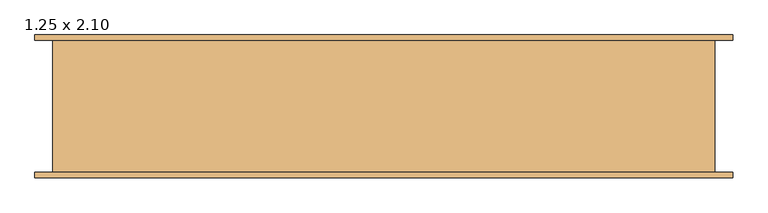
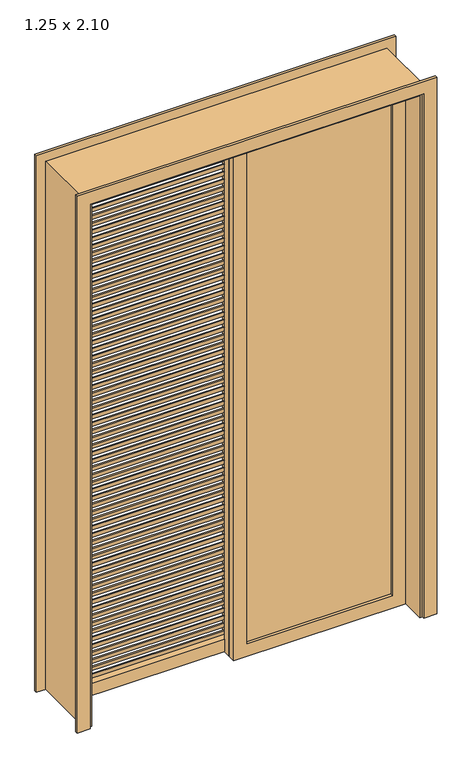
"""IFC4 building model written with IfcOpenShell, lengths in millimetres: door geometry, .CC_ND 300_PORTA DE CORRER_3 FOLHAS_VENEZIANA_VIDRO_COM EXTENSÃO : 1.25 x 2.10."""

import ifcopenshell
import ifcopenshell.guid

model = None  # the IFC model being written
_history = None  # IfcOwnerHistory: only IFC2X3 demands one
_inside = {}  # id of a spatial element -> (the spatial element, [elements in it])
_under = {}  # id of a project, library or spatial element -> (it, [spatial elements below it])
_declared = {}  # id of a project -> (the project, [libraries it declares])
_typed = {}  # id of a type object -> (the type object, [elements of that type])
_made_of = {}  # id of a material, layer set ... -> (it, [elements and type objects made of it])


def new_model(schema):
    """Start an empty IFC model of exactly this schema.

    Asked for "IFC4X3", IfcOpenShell would pick the latest addendum, in which some entities
    have other attributes; the version numbers below select the first issue.
    IFC2X3 requires an IfcOwnerHistory on every rooted entity: one is made here for all.
    """
    global model, _history
    if schema == "IFC4X3":
        model = ifcopenshell.file(schema_version=(4, 3, 0, 0))
    else:
        model = ifcopenshell.file(schema=schema)
    _inside.clear()
    _under.clear()
    _declared.clear()
    _typed.clear()
    _made_of.clear()
    _history = None
    if model.schema == "IFC2X3":
        org = make("IfcOrganization", Name="unknown")
        user = make(
            "IfcPersonAndOrganization",
            ThePerson=make("IfcPerson", FamilyName="unknown"),
            TheOrganization=org,
        )
        app = make(
            "IfcApplication",
            ApplicationDeveloper=org,
            Version="unknown",
            ApplicationFullName="unknown",
            ApplicationIdentifier="unknown",
        )
        _history = make(
            "IfcOwnerHistory",
            OwningUser=user,
            OwningApplication=app,
            ChangeAction="ADDED",
            CreationDate=0,
        )
    return model


def make(cls, **values):
    """One entity of the class cls with the attributes given. An attribute that is None is left unset."""
    return model.create_entity(
        cls, **{name: value for name, value in values.items() if value is not None}
    )


def rooted(cls, **values):
    """An entity with a GlobalId (a new one), such as an element, a storey or a relation."""
    return make(cls, GlobalId=ifcopenshell.guid.new(), OwnerHistory=_history, **values)


def si_unit(unit_type, name, prefix=None):
    """IfcSIUnit, for example si_unit("LENGTHUNIT", "METRE", prefix="MILLI")."""
    return make("IfcSIUnit", UnitType=unit_type, Prefix=prefix, Name=name)


def assignment(units):
    """IfcUnitAssignment: the units of a project."""
    return None if units is None else make("IfcUnitAssignment", Units=units)


def point(xyz):
    """IfcCartesianPoint."""
    return None if xyz is None else make("IfcCartesianPoint", Coordinates=xyz)


def direction(xyz):
    """IfcDirection."""
    return None if xyz is None else make("IfcDirection", DirectionRatios=xyz)


def frame(location, z_axis=None, x_axis=None):
    """IfcAxis2Placement3D, a coordinate frame: its origin and axes. An axis left out is left unset."""
    return make(
        "IfcAxis2Placement3D",
        Location=point(location),
        Axis=direction(z_axis),
        RefDirection=direction(x_axis),
    )


def origin():
    """The frame at (0, 0, 0) with its axes left unset."""
    return frame((0.0, 0.0, 0.0))


def place(relative_to, where):
    """IfcLocalPlacement: puts the frame where relative to a parent placement (None: the world)."""
    return make(
        "IfcLocalPlacement", PlacementRelTo=relative_to, RelativePlacement=where
    )


def context(
    kind, dimensions, precision=None, world=None, true_north=None, identifier=None
):
    """IfcGeometricRepresentationContext, for example the 3D "Model" context."""
    return make(
        "IfcGeometricRepresentationContext",
        ContextIdentifier=identifier,
        ContextType=kind,
        CoordinateSpaceDimension=dimensions,
        Precision=precision,
        WorldCoordinateSystem=world,
        TrueNorth=true_north,
    )


def project(units=None, contexts=None):
    """IfcProject with its units and contexts."""
    return rooted(
        "IfcProject",
        Name="project",
        RepresentationContexts=contexts,
        UnitsInContext=assignment(units),
    )


def spatial(cls, under=None, at=None, **own):
    """A site, building, storey or space (cls), placed at a placement, below another one or the project."""
    s = rooted(cls, ObjectPlacement=at, **own)
    if under is not None:
        _under.setdefault(under.id(), (under, []))[1].append(s)
    return s


def polyline(points):
    """IfcPolyline through the points."""
    return make("IfcPolyline", Points=[point(p) for p in points])


def outline(outer, holes=None, kind="AREA"):
    """IfcArbitraryClosedProfileDef: a profile drawn as a closed curve; with holes, ...WithVoids."""
    if holes is None:
        return make("IfcArbitraryClosedProfileDef", ProfileType=kind, OuterCurve=outer)
    return make(
        "IfcArbitraryProfileDefWithVoids",
        ProfileType=kind,
        OuterCurve=outer,
        InnerCurves=holes,
    )


def extrude(swept, where, along, depth):
    """IfcExtrudedAreaSolid: the profile swept, set in the frame where, extruded along a direction by depth."""
    return make(
        "IfcExtrudedAreaSolid",
        SweptArea=swept,
        Position=where,
        ExtrudedDirection=direction(along),
        Depth=depth,
    )


def shape(context_of_items, identifier, shape_type, items):
    """IfcShapeRepresentation: the items that make up one representation, for example the "Body"."""
    return make(
        "IfcShapeRepresentation",
        ContextOfItems=context_of_items,
        RepresentationIdentifier=identifier,
        RepresentationType=shape_type,
        Items=items,
    )


def source(mapping_origin, context_of_items, identifier, shape_type, items):
    """IfcRepresentationMap: a shape defined once, which mapped items show again and again."""
    return make(
        "IfcRepresentationMap",
        MappingOrigin=mapping_origin,
        MappedRepresentation=shape(context_of_items, identifier, shape_type, items),
    )


def transform(
    local_origin,
    x_axis=None,
    y_axis=None,
    z_axis=None,
    scale=None,
    scale2=None,
    scale3=None,
    uniform=True,
):
    """IfcCartesianTransformationOperator3D, or its non-uniform kind. x_axis, y_axis, z_axis: its Axis1, 2, 3."""
    if uniform:
        return make(
            "IfcCartesianTransformationOperator3D",
            Axis1=direction(x_axis),
            Axis2=direction(y_axis),
            LocalOrigin=point(local_origin),
            Scale=scale,
            Axis3=direction(z_axis),
        )
    return make(
        "IfcCartesianTransformationOperator3DnonUniform",
        Axis1=direction(x_axis),
        Axis2=direction(y_axis),
        LocalOrigin=point(local_origin),
        Scale=scale,
        Axis3=direction(z_axis),
        Scale2=scale2,
        Scale3=scale3,
    )


def mapped(mapping_source, mapping_target):
    """IfcMappedItem: shows the shape of a source again, moved by a transform."""
    return make(
        "IfcMappedItem", MappingSource=mapping_source, MappingTarget=mapping_target
    )


def made_of(thing, what):
    """Note that an element or type object is made of a material, layer set ...; save() writes the relation."""
    if what is not None:
        _made_of.setdefault(what.id(), (what, []))[1].append(thing)
    return thing


def element(
    cls,
    number,
    at=None,
    inside=None,
    cuts=None,
    type_object=None,
    material=None,
    context=None,
    identifier="Body",
    shape_type=None,
    held_by="IfcProductDefinitionShape",
    body=None,
    shapes=None,
    **own,
):
    """One element of the class cls, such as IfcWall. Its Tag is "e" and its number.

    at: its placement. inside: the storey or other place that contains it. cuts: it is an
    opening in that element (IfcRelVoidsElement). A single representation is given by context,
    identifier, shape_type and body (its items); several are given by shapes. held_by: the class
    of the entity that holds the representations. save() writes the other relations.
    """
    e = rooted(cls, Tag="e%d" % number, ObjectPlacement=at, **own)
    if body is not None:
        shapes = [shape(context, identifier, shape_type, body)]
    if shapes is not None:
        e.Representation = make(held_by, Representations=shapes)
    if inside is not None:
        _inside.setdefault(inside.id(), (inside, []))[1].append(e)
    if cuts is not None:
        rooted(
            "IfcRelVoidsElement", RelatingBuildingElement=cuts, RelatedOpeningElement=e
        )
    if type_object is not None:
        _typed.setdefault(type_object.id(), (type_object, []))[1].append(e)
    return made_of(e, material)


def aggregate(whole, parts):
    """IfcRelAggregates: a whole, such as a stair, and the parts it consists of."""
    return rooted("IfcRelAggregates", RelatingObject=whole, RelatedObjects=parts)


def save(model, path):
    """Write the relations noted so far, then the file.

    IfcRelAggregates (storeys below a building ...), IfcRelContainedInSpatialStructure (elements
    in a storey), IfcRelDefinesByType, IfcRelAssociatesMaterial and IfcRelDeclares: one each for
    every whole, place, type object, material and project.
    """
    for whole, parts in _under.values():
        aggregate(whole, parts)
    for where, things in _inside.values():
        rooted(
            "IfcRelContainedInSpatialStructure",
            RelatedElements=things,
            RelatingStructure=where,
        )
    for kind, things in _typed.values():
        rooted("IfcRelDefinesByType", RelatedObjects=things, RelatingType=kind)
    for what, things in _made_of.values():
        rooted("IfcRelAssociatesMaterial", RelatedObjects=things, RelatingMaterial=what)
    for by, libraries in _declared.values():
        rooted("IfcRelDeclares", RelatingContext=by, RelatedDefinitions=libraries)
    model.write(path)


def door_1_25_x_2_10_d20a60c6(model_context):
    return source(origin(), model_context, "Body", "SweptSolid", [
        extrude(outline(polyline([(575.0, -26.0), (575.0, -34.0), (20.0, -34.0), (20.0, -26.0), (575.0, -26.0)])), frame((0.0, 0.0, 50.0), z_axis=(0.0, 0.0, 1.0), x_axis=(1.0, 0.0, 0.0)), (0.0, 0.0, 1.0), 2000.0),
        extrude(outline(polyline([(2100.0, 625.0), (2100.0, -30.0), (0.0, -30.0), (0.0, 625.0), (2100.0, 625.0)]), holes=[polyline([(2050.0, 575.0), (50.0, 575.0), (50.0, 20.0), (2050.0, 20.0), (2050.0, 575.0)])]), frame((0.0, -45.0, 0.0), z_axis=(0.0, 1.0, 0.0), x_axis=(0.0, 0.0, 1.0)), (0.0, 0.0, 1.0), 30.0),
        extrude(outline(polyline([(40.0, 1985.2272727), (15.0, 2020.2272727), (20.0, 2020.2272727), (45.0, 1985.2272727), (40.0, 1985.2272727)])), frame((-575.0, 0.0, 0.0), z_axis=(1.0, 0.0, 0.0), x_axis=(0.0, 1.0, 0.0)), (0.0, 0.0, 1.0), 555.0),
        extrude(outline(polyline([(40.0, 1955.4545455), (15.0, 1990.4545455), (20.0, 1990.4545455), (45.0, 1955.4545455), (40.0, 1955.4545455)])), frame((-575.0, 0.0, 0.0), z_axis=(1.0, 0.0, 0.0), x_axis=(0.0, 1.0, 0.0)), (0.0, 0.0, 1.0), 555.0),
        extrude(outline(polyline([(40.0, 1925.6818182), (15.0, 1960.6818182), (20.0, 1960.6818182), (45.0, 1925.6818182), (40.0, 1925.6818182)])), frame((-575.0, 0.0, 0.0), z_axis=(1.0, 0.0, 0.0), x_axis=(0.0, 1.0, 0.0)), (0.0, 0.0, 1.0), 555.0),
        extrude(outline(polyline([(40.0, 1895.9090909), (15.0, 1930.9090909), (20.0, 1930.9090909), (45.0, 1895.9090909), (40.0, 1895.9090909)])), frame((-575.0, 0.0, 0.0), z_axis=(1.0, 0.0, 0.0), x_axis=(0.0, 1.0, 0.0)), (0.0, 0.0, 1.0), 555.0),
        extrude(outline(polyline([(40.0, 1866.1363636), (15.0, 1901.1363636), (20.0, 1901.1363636), (45.0, 1866.1363636), (40.0, 1866.1363636)])), frame((-575.0, 0.0, 0.0), z_axis=(1.0, 0.0, 0.0), x_axis=(0.0, 1.0, 0.0)), (0.0, 0.0, 1.0), 555.0),
        extrude(outline(polyline([(40.0, 1836.3636364), (15.0, 1871.3636364), (20.0, 1871.3636364), (45.0, 1836.3636364), (40.0, 1836.3636364)])), frame((-575.0, 0.0, 0.0), z_axis=(1.0, 0.0, 0.0), x_axis=(0.0, 1.0, 0.0)), (0.0, 0.0, 1.0), 555.0),
        extrude(outline(polyline([(40.0, 1806.5909091), (15.0, 1841.5909091), (20.0, 1841.5909091), (45.0, 1806.5909091), (40.0, 1806.5909091)])), frame((-575.0, 0.0, 0.0), z_axis=(1.0, 0.0, 0.0), x_axis=(0.0, 1.0, 0.0)), (0.0, 0.0, 1.0), 555.0),
        extrude(outline(polyline([(40.0, 1776.8181818), (15.0, 1811.8181818), (20.0, 1811.8181818), (45.0, 1776.8181818), (40.0, 1776.8181818)])), frame((-575.0, 0.0, 0.0), z_axis=(1.0, 0.0, 0.0), x_axis=(0.0, 1.0, 0.0)), (0.0, 0.0, 1.0), 555.0),
        extrude(outline(polyline([(40.0, 1747.0454545), (15.0, 1782.0454545), (20.0, 1782.0454545), (45.0, 1747.0454545), (40.0, 1747.0454545)])), frame((-575.0, 0.0, 0.0), z_axis=(1.0, 0.0, 0.0), x_axis=(0.0, 1.0, 0.0)), (0.0, 0.0, 1.0), 555.0),
        extrude(outline(polyline([(40.0, 1717.2727273), (15.0, 1752.2727273), (20.0, 1752.2727273), (45.0, 1717.2727273), (40.0, 1717.2727273)])), frame((-575.0, 0.0, 0.0), z_axis=(1.0, 0.0, 0.0), x_axis=(0.0, 1.0, 0.0)), (0.0, 0.0, 1.0), 555.0),
        extrude(outline(polyline([(40.0, 1687.5), (15.0, 1722.5), (20.0, 1722.5), (45.0, 1687.5), (40.0, 1687.5)])), frame((-575.0, 0.0, 0.0), z_axis=(1.0, 0.0, 0.0), x_axis=(0.0, 1.0, 0.0)), (0.0, 0.0, 1.0), 555.0),
        extrude(outline(polyline([(40.0, 1657.7272727), (15.0, 1692.7272727), (20.0, 1692.7272727), (45.0, 1657.7272727), (40.0, 1657.7272727)])), frame((-575.0, 0.0, 0.0), z_axis=(1.0, 0.0, 0.0), x_axis=(0.0, 1.0, 0.0)), (0.0, 0.0, 1.0), 555.0),
        extrude(outline(polyline([(40.0, 1627.9545455), (15.0, 1662.9545455), (20.0, 1662.9545455), (45.0, 1627.9545455), (40.0, 1627.9545455)])), frame((-575.0, 0.0, 0.0), z_axis=(1.0, 0.0, 0.0), x_axis=(0.0, 1.0, 0.0)), (0.0, 0.0, 1.0), 555.0),
        extrude(outline(polyline([(40.0, 1598.1818182), (15.0, 1633.1818182), (20.0, 1633.1818182), (45.0, 1598.1818182), (40.0, 1598.1818182)])), frame((-575.0, 0.0, 0.0), z_axis=(1.0, 0.0, 0.0), x_axis=(0.0, 1.0, 0.0)), (0.0, 0.0, 1.0), 555.0),
        extrude(outline(polyline([(40.0, 1568.4090909), (15.0, 1603.4090909), (20.0, 1603.4090909), (45.0, 1568.4090909), (40.0, 1568.4090909)])), frame((-575.0, 0.0, 0.0), z_axis=(1.0, 0.0, 0.0), x_axis=(0.0, 1.0, 0.0)), (0.0, 0.0, 1.0), 555.0),
        extrude(outline(polyline([(40.0, 1538.6363636), (15.0, 1573.6363636), (20.0, 1573.6363636), (45.0, 1538.6363636), (40.0, 1538.6363636)])), frame((-575.0, 0.0, 0.0), z_axis=(1.0, 0.0, 0.0), x_axis=(0.0, 1.0, 0.0)), (0.0, 0.0, 1.0), 555.0),
        extrude(outline(polyline([(40.0, 1508.8636364), (15.0, 1543.8636364), (20.0, 1543.8636364), (45.0, 1508.8636364), (40.0, 1508.8636364)])), frame((-575.0, 0.0, 0.0), z_axis=(1.0, 0.0, 0.0), x_axis=(0.0, 1.0, 0.0)), (0.0, 0.0, 1.0), 555.0),
        extrude(outline(polyline([(40.0, 1479.0909091), (15.0, 1514.0909091), (20.0, 1514.0909091), (45.0, 1479.0909091), (40.0, 1479.0909091)])), frame((-575.0, 0.0, 0.0), z_axis=(1.0, 0.0, 0.0), x_axis=(0.0, 1.0, 0.0)), (0.0, 0.0, 1.0), 555.0),
        extrude(outline(polyline([(40.0, 1449.3181818), (15.0, 1484.3181818), (20.0, 1484.3181818), (45.0, 1449.3181818), (40.0, 1449.3181818)])), frame((-575.0, 0.0, 0.0), z_axis=(1.0, 0.0, 0.0), x_axis=(0.0, 1.0, 0.0)), (0.0, 0.0, 1.0), 555.0),
        extrude(outline(polyline([(40.0, 1419.5454545), (15.0, 1454.5454545), (20.0, 1454.5454545), (45.0, 1419.5454545), (40.0, 1419.5454545)])), frame((-575.0, 0.0, 0.0), z_axis=(1.0, 0.0, 0.0), x_axis=(0.0, 1.0, 0.0)), (0.0, 0.0, 1.0), 555.0),
        extrude(outline(polyline([(40.0, 1389.7727273), (15.0, 1424.7727273), (20.0, 1424.7727273), (45.0, 1389.7727273), (40.0, 1389.7727273)])), frame((-575.0, 0.0, 0.0), z_axis=(1.0, 0.0, 0.0), x_axis=(0.0, 1.0, 0.0)), (0.0, 0.0, 1.0), 555.0),
        extrude(outline(polyline([(40.0, 1360.0), (15.0, 1395.0), (20.0, 1395.0), (45.0, 1360.0), (40.0, 1360.0)])), frame((-575.0, 0.0, 0.0), z_axis=(1.0, 0.0, 0.0), x_axis=(0.0, 1.0, 0.0)), (0.0, 0.0, 1.0), 555.0),
        extrude(outline(polyline([(40.0, 1330.2272727), (15.0, 1365.2272727), (20.0, 1365.2272727), (45.0, 1330.2272727), (40.0, 1330.2272727)])), frame((-575.0, 0.0, 0.0), z_axis=(1.0, 0.0, 0.0), x_axis=(0.0, 1.0, 0.0)), (0.0, 0.0, 1.0), 555.0),
        extrude(outline(polyline([(40.0, 1300.4545455), (15.0, 1335.4545455), (20.0, 1335.4545455), (45.0, 1300.4545455), (40.0, 1300.4545455)])), frame((-575.0, 0.0, 0.0), z_axis=(1.0, 0.0, 0.0), x_axis=(0.0, 1.0, 0.0)), (0.0, 0.0, 1.0), 555.0),
        extrude(outline(polyline([(40.0, 1270.6818182), (15.0, 1305.6818182), (20.0, 1305.6818182), (45.0, 1270.6818182), (40.0, 1270.6818182)])), frame((-575.0, 0.0, 0.0), z_axis=(1.0, 0.0, 0.0), x_axis=(0.0, 1.0, 0.0)), (0.0, 0.0, 1.0), 555.0),
        extrude(outline(polyline([(40.0, 1240.9090909), (15.0, 1275.9090909), (20.0, 1275.9090909), (45.0, 1240.9090909), (40.0, 1240.9090909)])), frame((-575.0, 0.0, 0.0), z_axis=(1.0, 0.0, 0.0), x_axis=(0.0, 1.0, 0.0)), (0.0, 0.0, 1.0), 555.0),
        extrude(outline(polyline([(40.0, 1211.1363636), (15.0, 1246.1363636), (20.0, 1246.1363636), (45.0, 1211.1363636), (40.0, 1211.1363636)])), frame((-575.0, 0.0, 0.0), z_axis=(1.0, 0.0, 0.0), x_axis=(0.0, 1.0, 0.0)), (0.0, 0.0, 1.0), 555.0),
        extrude(outline(polyline([(40.0, 1181.3636364), (15.0, 1216.3636364), (20.0, 1216.3636364), (45.0, 1181.3636364), (40.0, 1181.3636364)])), frame((-575.0, 0.0, 0.0), z_axis=(1.0, 0.0, 0.0), x_axis=(0.0, 1.0, 0.0)), (0.0, 0.0, 1.0), 555.0),
        extrude(outline(polyline([(40.0, 1151.5909091), (15.0, 1186.5909091), (20.0, 1186.5909091), (45.0, 1151.5909091), (40.0, 1151.5909091)])), frame((-575.0, 0.0, 0.0), z_axis=(1.0, 0.0, 0.0), x_axis=(0.0, 1.0, 0.0)), (0.0, 0.0, 1.0), 555.0),
        extrude(outline(polyline([(40.0, 1121.8181818), (15.0, 1156.8181818), (20.0, 1156.8181818), (45.0, 1121.8181818), (40.0, 1121.8181818)])), frame((-575.0, 0.0, 0.0), z_axis=(1.0, 0.0, 0.0), x_axis=(0.0, 1.0, 0.0)), (0.0, 0.0, 1.0), 555.0),
        extrude(outline(polyline([(40.0, 1092.0454545), (15.0, 1127.0454545), (20.0, 1127.0454545), (45.0, 1092.0454545), (40.0, 1092.0454545)])), frame((-575.0, 0.0, 0.0), z_axis=(1.0, 0.0, 0.0), x_axis=(0.0, 1.0, 0.0)), (0.0, 0.0, 1.0), 555.0),
        extrude(outline(polyline([(40.0, 1062.2727273), (15.0, 1097.2727273), (20.0, 1097.2727273), (45.0, 1062.2727273), (40.0, 1062.2727273)])), frame((-575.0, 0.0, 0.0), z_axis=(1.0, 0.0, 0.0), x_axis=(0.0, 1.0, 0.0)), (0.0, 0.0, 1.0), 555.0),
        extrude(outline(polyline([(40.0, 1032.5), (15.0, 1067.5), (20.0, 1067.5), (45.0, 1032.5), (40.0, 1032.5)])), frame((-575.0, 0.0, 0.0), z_axis=(1.0, 0.0, 0.0), x_axis=(0.0, 1.0, 0.0)), (0.0, 0.0, 1.0), 555.0),
        extrude(outline(polyline([(40.0, 1002.7272727), (15.0, 1037.7272727), (20.0, 1037.7272727), (45.0, 1002.7272727), (40.0, 1002.7272727)])), frame((-575.0, 0.0, 0.0), z_axis=(1.0, 0.0, 0.0), x_axis=(0.0, 1.0, 0.0)), (0.0, 0.0, 1.0), 555.0),
        extrude(outline(polyline([(40.0, 972.9545455), (15.0, 1007.9545455), (20.0, 1007.9545455), (45.0, 972.9545455), (40.0, 972.9545455)])), frame((-575.0, 0.0, 0.0), z_axis=(1.0, 0.0, 0.0), x_axis=(0.0, 1.0, 0.0)), (0.0, 0.0, 1.0), 555.0),
        extrude(outline(polyline([(40.0, 943.1818182), (15.0, 978.1818182), (20.0, 978.1818182), (45.0, 943.1818182), (40.0, 943.1818182)])), frame((-575.0, 0.0, 0.0), z_axis=(1.0, 0.0, 0.0), x_axis=(0.0, 1.0, 0.0)), (0.0, 0.0, 1.0), 555.0),
        extrude(outline(polyline([(40.0, 913.4090909), (15.0, 948.4090909), (20.0, 948.4090909), (45.0, 913.4090909), (40.0, 913.4090909)])), frame((-575.0, 0.0, 0.0), z_axis=(1.0, 0.0, 0.0), x_axis=(0.0, 1.0, 0.0)), (0.0, 0.0, 1.0), 555.0),
        extrude(outline(polyline([(40.0, 883.6363636), (15.0, 918.6363636), (20.0, 918.6363636), (45.0, 883.6363636), (40.0, 883.6363636)])), frame((-575.0, 0.0, 0.0), z_axis=(1.0, 0.0, 0.0), x_axis=(0.0, 1.0, 0.0)), (0.0, 0.0, 1.0), 555.0),
        extrude(outline(polyline([(40.0, 853.8636364), (15.0, 888.8636364), (20.0, 888.8636364), (45.0, 853.8636364), (40.0, 853.8636364)])), frame((-575.0, 0.0, 0.0), z_axis=(1.0, 0.0, 0.0), x_axis=(0.0, 1.0, 0.0)), (0.0, 0.0, 1.0), 555.0),
        extrude(outline(polyline([(40.0, 824.0909091), (15.0, 859.0909091), (20.0, 859.0909091), (45.0, 824.0909091), (40.0, 824.0909091)])), frame((-575.0, 0.0, 0.0), z_axis=(1.0, 0.0, 0.0), x_axis=(0.0, 1.0, 0.0)), (0.0, 0.0, 1.0), 555.0),
        extrude(outline(polyline([(40.0, 794.3181818), (15.0, 829.3181818), (20.0, 829.3181818), (45.0, 794.3181818), (40.0, 794.3181818)])), frame((-575.0, 0.0, 0.0), z_axis=(1.0, 0.0, 0.0), x_axis=(0.0, 1.0, 0.0)), (0.0, 0.0, 1.0), 555.0),
        extrude(outline(polyline([(40.0, 764.5454545), (15.0, 799.5454545), (20.0, 799.5454545), (45.0, 764.5454545), (40.0, 764.5454545)])), frame((-575.0, 0.0, 0.0), z_axis=(1.0, 0.0, 0.0), x_axis=(0.0, 1.0, 0.0)), (0.0, 0.0, 1.0), 555.0),
        extrude(outline(polyline([(40.0, 734.7727273), (15.0, 769.7727273), (20.0, 769.7727273), (45.0, 734.7727273), (40.0, 734.7727273)])), frame((-575.0, 0.0, 0.0), z_axis=(1.0, 0.0, 0.0), x_axis=(0.0, 1.0, 0.0)), (0.0, 0.0, 1.0), 555.0),
        extrude(outline(polyline([(40.0, 705.0), (15.0, 740.0), (20.0, 740.0), (45.0, 705.0), (40.0, 705.0)])), frame((-575.0, 0.0, 0.0), z_axis=(1.0, 0.0, 0.0), x_axis=(0.0, 1.0, 0.0)), (0.0, 0.0, 1.0), 555.0),
        extrude(outline(polyline([(40.0, 675.2272727), (15.0, 710.2272727), (20.0, 710.2272727), (45.0, 675.2272727), (40.0, 675.2272727)])), frame((-575.0, 0.0, 0.0), z_axis=(1.0, 0.0, 0.0), x_axis=(0.0, 1.0, 0.0)), (0.0, 0.0, 1.0), 555.0),
        extrude(outline(polyline([(40.0, 645.4545455), (15.0, 680.4545455), (20.0, 680.4545455), (45.0, 645.4545455), (40.0, 645.4545455)])), frame((-575.0, 0.0, 0.0), z_axis=(1.0, 0.0, 0.0), x_axis=(0.0, 1.0, 0.0)), (0.0, 0.0, 1.0), 555.0),
        extrude(outline(polyline([(40.0, 615.6818182), (15.0, 650.6818182), (20.0, 650.6818182), (45.0, 615.6818182), (40.0, 615.6818182)])), frame((-575.0, 0.0, 0.0), z_axis=(1.0, 0.0, 0.0), x_axis=(0.0, 1.0, 0.0)), (0.0, 0.0, 1.0), 555.0),
        extrude(outline(polyline([(40.0, 585.9090909), (15.0, 620.9090909), (20.0, 620.9090909), (45.0, 585.9090909), (40.0, 585.9090909)])), frame((-575.0, 0.0, 0.0), z_axis=(1.0, 0.0, 0.0), x_axis=(0.0, 1.0, 0.0)), (0.0, 0.0, 1.0), 555.0),
        extrude(outline(polyline([(40.0, 556.1363636), (15.0, 591.1363636), (20.0, 591.1363636), (45.0, 556.1363636), (40.0, 556.1363636)])), frame((-575.0, 0.0, 0.0), z_axis=(1.0, 0.0, 0.0), x_axis=(0.0, 1.0, 0.0)), (0.0, 0.0, 1.0), 555.0),
        extrude(outline(polyline([(40.0, 526.3636364), (15.0, 561.3636364), (20.0, 561.3636364), (45.0, 526.3636364), (40.0, 526.3636364)])), frame((-575.0, 0.0, 0.0), z_axis=(1.0, 0.0, 0.0), x_axis=(0.0, 1.0, 0.0)), (0.0, 0.0, 1.0), 555.0),
        extrude(outline(polyline([(40.0, 496.5909091), (15.0, 531.5909091), (20.0, 531.5909091), (45.0, 496.5909091), (40.0, 496.5909091)])), frame((-575.0, 0.0, 0.0), z_axis=(1.0, 0.0, 0.0), x_axis=(0.0, 1.0, 0.0)), (0.0, 0.0, 1.0), 555.0),
        extrude(outline(polyline([(40.0, 466.8181818), (15.0, 501.8181818), (20.0, 501.8181818), (45.0, 466.8181818), (40.0, 466.8181818)])), frame((-575.0, 0.0, 0.0), z_axis=(1.0, 0.0, 0.0), x_axis=(0.0, 1.0, 0.0)), (0.0, 0.0, 1.0), 555.0),
        extrude(outline(polyline([(40.0, 437.0454545), (15.0, 472.0454545), (20.0, 472.0454545), (45.0, 437.0454545), (40.0, 437.0454545)])), frame((-575.0, 0.0, 0.0), z_axis=(1.0, 0.0, 0.0), x_axis=(0.0, 1.0, 0.0)), (0.0, 0.0, 1.0), 555.0),
        extrude(outline(polyline([(40.0, 407.2727273), (15.0, 442.2727273), (20.0, 442.2727273), (45.0, 407.2727273), (40.0, 407.2727273)])), frame((-575.0, 0.0, 0.0), z_axis=(1.0, 0.0, 0.0), x_axis=(0.0, 1.0, 0.0)), (0.0, 0.0, 1.0), 555.0),
        extrude(outline(polyline([(40.0, 377.5), (15.0, 412.5), (20.0, 412.5), (45.0, 377.5), (40.0, 377.5)])), frame((-575.0, 0.0, 0.0), z_axis=(1.0, 0.0, 0.0), x_axis=(0.0, 1.0, 0.0)), (0.0, 0.0, 1.0), 555.0),
        extrude(outline(polyline([(40.0, 347.7272727), (15.0, 382.7272727), (20.0, 382.7272727), (45.0, 347.7272727), (40.0, 347.7272727)])), frame((-575.0, 0.0, 0.0), z_axis=(1.0, 0.0, 0.0), x_axis=(0.0, 1.0, 0.0)), (0.0, 0.0, 1.0), 555.0),
        extrude(outline(polyline([(40.0, 317.9545455), (15.0, 352.9545455), (20.0, 352.9545455), (45.0, 317.9545455), (40.0, 317.9545455)])), frame((-575.0, 0.0, 0.0), z_axis=(1.0, 0.0, 0.0), x_axis=(0.0, 1.0, 0.0)), (0.0, 0.0, 1.0), 555.0),
        extrude(outline(polyline([(40.0, 288.1818182), (15.0, 323.1818182), (20.0, 323.1818182), (45.0, 288.1818182), (40.0, 288.1818182)])), frame((-575.0, 0.0, 0.0), z_axis=(1.0, 0.0, 0.0), x_axis=(0.0, 1.0, 0.0)), (0.0, 0.0, 1.0), 555.0),
        extrude(outline(polyline([(40.0, 258.4090909), (15.0, 293.4090909), (20.0, 293.4090909), (45.0, 258.4090909), (40.0, 258.4090909)])), frame((-575.0, 0.0, 0.0), z_axis=(1.0, 0.0, 0.0), x_axis=(0.0, 1.0, 0.0)), (0.0, 0.0, 1.0), 555.0),
        extrude(outline(polyline([(40.0, 228.6363636), (15.0, 263.6363636), (20.0, 263.6363636), (45.0, 228.6363636), (40.0, 228.6363636)])), frame((-575.0, 0.0, 0.0), z_axis=(1.0, 0.0, 0.0), x_axis=(0.0, 1.0, 0.0)), (0.0, 0.0, 1.0), 555.0),
        extrude(outline(polyline([(40.0, 198.8636364), (15.0, 233.8636364), (20.0, 233.8636364), (45.0, 198.8636364), (40.0, 198.8636364)])), frame((-575.0, 0.0, 0.0), z_axis=(1.0, 0.0, 0.0), x_axis=(0.0, 1.0, 0.0)), (0.0, 0.0, 1.0), 555.0),
        extrude(outline(polyline([(40.0, 169.0909091), (15.0, 204.0909091), (20.0, 204.0909091), (45.0, 169.0909091), (40.0, 169.0909091)])), frame((-575.0, 0.0, 0.0), z_axis=(1.0, 0.0, 0.0), x_axis=(0.0, 1.0, 0.0)), (0.0, 0.0, 1.0), 555.0),
        extrude(outline(polyline([(40.0, 139.3181818), (15.0, 174.3181818), (20.0, 174.3181818), (45.0, 139.3181818), (40.0, 139.3181818)])), frame((-575.0, 0.0, 0.0), z_axis=(1.0, 0.0, 0.0), x_axis=(0.0, 1.0, 0.0)), (0.0, 0.0, 1.0), 555.0),
        extrude(outline(polyline([(40.0, 109.5454545), (15.0, 144.5454545), (20.0, 144.5454545), (45.0, 109.5454545), (40.0, 109.5454545)])), frame((-575.0, 0.0, 0.0), z_axis=(1.0, 0.0, 0.0), x_axis=(0.0, 1.0, 0.0)), (0.0, 0.0, 1.0), 555.0),
        extrude(outline(polyline([(40.0, 79.7727273), (15.0, 114.7727273), (20.0, 114.7727273), (45.0, 79.7727273), (40.0, 79.7727273)])), frame((-575.0, 0.0, 0.0), z_axis=(1.0, 0.0, 0.0), x_axis=(0.0, 1.0, 0.0)), (0.0, 0.0, 1.0), 555.0),
        extrude(outline(polyline([(40.0, 2015.0), (15.0, 2050.0), (20.0, 2050.0), (45.0, 2015.0), (40.0, 2015.0)])), frame((-575.0, 0.0, 0.0), z_axis=(1.0, 0.0, 0.0), x_axis=(0.0, 1.0, 0.0)), (0.0, 0.0, 1.0), 555.0),
        extrude(outline(polyline([(40.0, 50.0), (15.0, 85.0), (20.0, 85.0), (45.0, 50.0), (40.0, 50.0)])), frame((-575.0, 0.0, 0.0), z_axis=(1.0, 0.0, 0.0), x_axis=(0.0, 1.0, 0.0)), (0.0, 0.0, 1.0), 555.0),
        extrude(outline(polyline([(2100.0, 30.0), (2100.0, -625.0), (0.0, -625.0), (0.0, 30.0), (2100.0, 30.0)]), holes=[polyline([(2050.0, -20.0), (50.0, -20.0), (50.0, -575.0), (2050.0, -575.0), (2050.0, -20.0)])]), frame((0.0, 15.0, 0.0), z_axis=(0.0, 1.0, 0.0), x_axis=(0.0, 0.0, 1.0)), (0.0, 0.0, 1.0), 30.0),
        extrude(outline(polyline([(10.0, 1985.2272727), (-15.0, 2020.2272727), (-10.0, 2020.2272727), (15.0, 1985.2272727), (10.0, 1985.2272727)])), frame((20.0, 0.0, 0.0), z_axis=(1.0, 0.0, 0.0), x_axis=(0.0, 1.0, 0.0)), (0.0, 0.0, 1.0), 555.0),
        extrude(outline(polyline([(10.0, 1955.4545455), (-15.0, 1990.4545455), (-10.0, 1990.4545455), (15.0, 1955.4545455), (10.0, 1955.4545455)])), frame((20.0, 0.0, 0.0), z_axis=(1.0, 0.0, 0.0), x_axis=(0.0, 1.0, 0.0)), (0.0, 0.0, 1.0), 555.0),
        extrude(outline(polyline([(10.0, 1925.6818182), (-15.0, 1960.6818182), (-10.0, 1960.6818182), (15.0, 1925.6818182), (10.0, 1925.6818182)])), frame((20.0, 0.0, 0.0), z_axis=(1.0, 0.0, 0.0), x_axis=(0.0, 1.0, 0.0)), (0.0, 0.0, 1.0), 555.0),
        extrude(outline(polyline([(10.0, 1895.9090909), (-15.0, 1930.9090909), (-10.0, 1930.9090909), (15.0, 1895.9090909), (10.0, 1895.9090909)])), frame((20.0, 0.0, 0.0), z_axis=(1.0, 0.0, 0.0), x_axis=(0.0, 1.0, 0.0)), (0.0, 0.0, 1.0), 555.0),
        extrude(outline(polyline([(10.0, 1866.1363636), (-15.0, 1901.1363636), (-10.0, 1901.1363636), (15.0, 1866.1363636), (10.0, 1866.1363636)])), frame((20.0, 0.0, 0.0), z_axis=(1.0, 0.0, 0.0), x_axis=(0.0, 1.0, 0.0)), (0.0, 0.0, 1.0), 555.0),
        extrude(outline(polyline([(10.0, 1836.3636364), (-15.0, 1871.3636364), (-10.0, 1871.3636364), (15.0, 1836.3636364), (10.0, 1836.3636364)])), frame((20.0, 0.0, 0.0), z_axis=(1.0, 0.0, 0.0), x_axis=(0.0, 1.0, 0.0)), (0.0, 0.0, 1.0), 555.0),
        extrude(outline(polyline([(10.0, 1806.5909091), (-15.0, 1841.5909091), (-10.0, 1841.5909091), (15.0, 1806.5909091), (10.0, 1806.5909091)])), frame((20.0, 0.0, 0.0), z_axis=(1.0, 0.0, 0.0), x_axis=(0.0, 1.0, 0.0)), (0.0, 0.0, 1.0), 555.0),
        extrude(outline(polyline([(10.0, 1776.8181818), (-15.0, 1811.8181818), (-10.0, 1811.8181818), (15.0, 1776.8181818), (10.0, 1776.8181818)])), frame((20.0, 0.0, 0.0), z_axis=(1.0, 0.0, 0.0), x_axis=(0.0, 1.0, 0.0)), (0.0, 0.0, 1.0), 555.0),
        extrude(outline(polyline([(10.0, 1747.0454545), (-15.0, 1782.0454545), (-10.0, 1782.0454545), (15.0, 1747.0454545), (10.0, 1747.0454545)])), frame((20.0, 0.0, 0.0), z_axis=(1.0, 0.0, 0.0), x_axis=(0.0, 1.0, 0.0)), (0.0, 0.0, 1.0), 555.0),
        extrude(outline(polyline([(10.0, 1717.2727273), (-15.0, 1752.2727273), (-10.0, 1752.2727273), (15.0, 1717.2727273), (10.0, 1717.2727273)])), frame((20.0, 0.0, 0.0), z_axis=(1.0, 0.0, 0.0), x_axis=(0.0, 1.0, 0.0)), (0.0, 0.0, 1.0), 555.0),
        extrude(outline(polyline([(10.0, 1687.5), (-15.0, 1722.5), (-10.0, 1722.5), (15.0, 1687.5), (10.0, 1687.5)])), frame((20.0, 0.0, 0.0), z_axis=(1.0, 0.0, 0.0), x_axis=(0.0, 1.0, 0.0)), (0.0, 0.0, 1.0), 555.0),
        extrude(outline(polyline([(10.0, 1657.7272727), (-15.0, 1692.7272727), (-10.0, 1692.7272727), (15.0, 1657.7272727), (10.0, 1657.7272727)])), frame((20.0, 0.0, 0.0), z_axis=(1.0, 0.0, 0.0), x_axis=(0.0, 1.0, 0.0)), (0.0, 0.0, 1.0), 555.0),
        extrude(outline(polyline([(10.0, 1627.9545455), (-15.0, 1662.9545455), (-10.0, 1662.9545455), (15.0, 1627.9545455), (10.0, 1627.9545455)])), frame((20.0, 0.0, 0.0), z_axis=(1.0, 0.0, 0.0), x_axis=(0.0, 1.0, 0.0)), (0.0, 0.0, 1.0), 555.0),
        extrude(outline(polyline([(10.0, 1598.1818182), (-15.0, 1633.1818182), (-10.0, 1633.1818182), (15.0, 1598.1818182), (10.0, 1598.1818182)])), frame((20.0, 0.0, 0.0), z_axis=(1.0, 0.0, 0.0), x_axis=(0.0, 1.0, 0.0)), (0.0, 0.0, 1.0), 555.0),
        extrude(outline(polyline([(10.0, 1568.4090909), (-15.0, 1603.4090909), (-10.0, 1603.4090909), (15.0, 1568.4090909), (10.0, 1568.4090909)])), frame((20.0, 0.0, 0.0), z_axis=(1.0, 0.0, 0.0), x_axis=(0.0, 1.0, 0.0)), (0.0, 0.0, 1.0), 555.0),
        extrude(outline(polyline([(10.0, 1538.6363636), (-15.0, 1573.6363636), (-10.0, 1573.6363636), (15.0, 1538.6363636), (10.0, 1538.6363636)])), frame((20.0, 0.0, 0.0), z_axis=(1.0, 0.0, 0.0), x_axis=(0.0, 1.0, 0.0)), (0.0, 0.0, 1.0), 555.0),
        extrude(outline(polyline([(10.0, 1508.8636364), (-15.0, 1543.8636364), (-10.0, 1543.8636364), (15.0, 1508.8636364), (10.0, 1508.8636364)])), frame((20.0, 0.0, 0.0), z_axis=(1.0, 0.0, 0.0), x_axis=(0.0, 1.0, 0.0)), (0.0, 0.0, 1.0), 555.0),
        extrude(outline(polyline([(10.0, 1479.0909091), (-15.0, 1514.0909091), (-10.0, 1514.0909091), (15.0, 1479.0909091), (10.0, 1479.0909091)])), frame((20.0, 0.0, 0.0), z_axis=(1.0, 0.0, 0.0), x_axis=(0.0, 1.0, 0.0)), (0.0, 0.0, 1.0), 555.0),
        extrude(outline(polyline([(10.0, 1449.3181818), (-15.0, 1484.3181818), (-10.0, 1484.3181818), (15.0, 1449.3181818), (10.0, 1449.3181818)])), frame((20.0, 0.0, 0.0), z_axis=(1.0, 0.0, 0.0), x_axis=(0.0, 1.0, 0.0)), (0.0, 0.0, 1.0), 555.0),
        extrude(outline(polyline([(10.0, 1419.5454545), (-15.0, 1454.5454545), (-10.0, 1454.5454545), (15.0, 1419.5454545), (10.0, 1419.5454545)])), frame((20.0, 0.0, 0.0), z_axis=(1.0, 0.0, 0.0), x_axis=(0.0, 1.0, 0.0)), (0.0, 0.0, 1.0), 555.0),
        extrude(outline(polyline([(10.0, 1389.7727273), (-15.0, 1424.7727273), (-10.0, 1424.7727273), (15.0, 1389.7727273), (10.0, 1389.7727273)])), frame((20.0, 0.0, 0.0), z_axis=(1.0, 0.0, 0.0), x_axis=(0.0, 1.0, 0.0)), (0.0, 0.0, 1.0), 555.0),
        extrude(outline(polyline([(10.0, 1360.0), (-15.0, 1395.0), (-10.0, 1395.0), (15.0, 1360.0), (10.0, 1360.0)])), frame((20.0, 0.0, 0.0), z_axis=(1.0, 0.0, 0.0), x_axis=(0.0, 1.0, 0.0)), (0.0, 0.0, 1.0), 555.0),
        extrude(outline(polyline([(10.0, 1330.2272727), (-15.0, 1365.2272727), (-10.0, 1365.2272727), (15.0, 1330.2272727), (10.0, 1330.2272727)])), frame((20.0, 0.0, 0.0), z_axis=(1.0, 0.0, 0.0), x_axis=(0.0, 1.0, 0.0)), (0.0, 0.0, 1.0), 555.0),
        extrude(outline(polyline([(10.0, 1300.4545455), (-15.0, 1335.4545455), (-10.0, 1335.4545455), (15.0, 1300.4545455), (10.0, 1300.4545455)])), frame((20.0, 0.0, 0.0), z_axis=(1.0, 0.0, 0.0), x_axis=(0.0, 1.0, 0.0)), (0.0, 0.0, 1.0), 555.0),
        extrude(outline(polyline([(10.0, 1270.6818182), (-15.0, 1305.6818182), (-10.0, 1305.6818182), (15.0, 1270.6818182), (10.0, 1270.6818182)])), frame((20.0, 0.0, 0.0), z_axis=(1.0, 0.0, 0.0), x_axis=(0.0, 1.0, 0.0)), (0.0, 0.0, 1.0), 555.0),
        extrude(outline(polyline([(10.0, 1240.9090909), (-15.0, 1275.9090909), (-10.0, 1275.9090909), (15.0, 1240.9090909), (10.0, 1240.9090909)])), frame((20.0, 0.0, 0.0), z_axis=(1.0, 0.0, 0.0), x_axis=(0.0, 1.0, 0.0)), (0.0, 0.0, 1.0), 555.0),
        extrude(outline(polyline([(10.0, 1211.1363636), (-15.0, 1246.1363636), (-10.0, 1246.1363636), (15.0, 1211.1363636), (10.0, 1211.1363636)])), frame((20.0, 0.0, 0.0), z_axis=(1.0, 0.0, 0.0), x_axis=(0.0, 1.0, 0.0)), (0.0, 0.0, 1.0), 555.0),
        extrude(outline(polyline([(10.0, 1181.3636364), (-15.0, 1216.3636364), (-10.0, 1216.3636364), (15.0, 1181.3636364), (10.0, 1181.3636364)])), frame((20.0, 0.0, 0.0), z_axis=(1.0, 0.0, 0.0), x_axis=(0.0, 1.0, 0.0)), (0.0, 0.0, 1.0), 555.0),
        extrude(outline(polyline([(10.0, 1151.5909091), (-15.0, 1186.5909091), (-10.0, 1186.5909091), (15.0, 1151.5909091), (10.0, 1151.5909091)])), frame((20.0, 0.0, 0.0), z_axis=(1.0, 0.0, 0.0), x_axis=(0.0, 1.0, 0.0)), (0.0, 0.0, 1.0), 555.0),
        extrude(outline(polyline([(10.0, 1121.8181818), (-15.0, 1156.8181818), (-10.0, 1156.8181818), (15.0, 1121.8181818), (10.0, 1121.8181818)])), frame((20.0, 0.0, 0.0), z_axis=(1.0, 0.0, 0.0), x_axis=(0.0, 1.0, 0.0)), (0.0, 0.0, 1.0), 555.0),
        extrude(outline(polyline([(10.0, 1092.0454545), (-15.0, 1127.0454545), (-10.0, 1127.0454545), (15.0, 1092.0454545), (10.0, 1092.0454545)])), frame((20.0, 0.0, 0.0), z_axis=(1.0, 0.0, 0.0), x_axis=(0.0, 1.0, 0.0)), (0.0, 0.0, 1.0), 555.0),
        extrude(outline(polyline([(10.0, 1062.2727273), (-15.0, 1097.2727273), (-10.0, 1097.2727273), (15.0, 1062.2727273), (10.0, 1062.2727273)])), frame((20.0, 0.0, 0.0), z_axis=(1.0, 0.0, 0.0), x_axis=(0.0, 1.0, 0.0)), (0.0, 0.0, 1.0), 555.0),
        extrude(outline(polyline([(10.0, 1032.5), (-15.0, 1067.5), (-10.0, 1067.5), (15.0, 1032.5), (10.0, 1032.5)])), frame((20.0, 0.0, 0.0), z_axis=(1.0, 0.0, 0.0), x_axis=(0.0, 1.0, 0.0)), (0.0, 0.0, 1.0), 555.0),
        extrude(outline(polyline([(10.0, 1002.7272727), (-15.0, 1037.7272727), (-10.0, 1037.7272727), (15.0, 1002.7272727), (10.0, 1002.7272727)])), frame((20.0, 0.0, 0.0), z_axis=(1.0, 0.0, 0.0), x_axis=(0.0, 1.0, 0.0)), (0.0, 0.0, 1.0), 555.0),
        extrude(outline(polyline([(10.0, 972.9545455), (-15.0, 1007.9545455), (-10.0, 1007.9545455), (15.0, 972.9545455), (10.0, 972.9545455)])), frame((20.0, 0.0, 0.0), z_axis=(1.0, 0.0, 0.0), x_axis=(0.0, 1.0, 0.0)), (0.0, 0.0, 1.0), 555.0),
        extrude(outline(polyline([(10.0, 943.1818182), (-15.0, 978.1818182), (-10.0, 978.1818182), (15.0, 943.1818182), (10.0, 943.1818182)])), frame((20.0, 0.0, 0.0), z_axis=(1.0, 0.0, 0.0), x_axis=(0.0, 1.0, 0.0)), (0.0, 0.0, 1.0), 555.0),
        extrude(outline(polyline([(10.0, 913.4090909), (-15.0, 948.4090909), (-10.0, 948.4090909), (15.0, 913.4090909), (10.0, 913.4090909)])), frame((20.0, 0.0, 0.0), z_axis=(1.0, 0.0, 0.0), x_axis=(0.0, 1.0, 0.0)), (0.0, 0.0, 1.0), 555.0),
        extrude(outline(polyline([(10.0, 883.6363636), (-15.0, 918.6363636), (-10.0, 918.6363636), (15.0, 883.6363636), (10.0, 883.6363636)])), frame((20.0, 0.0, 0.0), z_axis=(1.0, 0.0, 0.0), x_axis=(0.0, 1.0, 0.0)), (0.0, 0.0, 1.0), 555.0),
        extrude(outline(polyline([(10.0, 853.8636364), (-15.0, 888.8636364), (-10.0, 888.8636364), (15.0, 853.8636364), (10.0, 853.8636364)])), frame((20.0, 0.0, 0.0), z_axis=(1.0, 0.0, 0.0), x_axis=(0.0, 1.0, 0.0)), (0.0, 0.0, 1.0), 555.0),
        extrude(outline(polyline([(10.0, 824.0909091), (-15.0, 859.0909091), (-10.0, 859.0909091), (15.0, 824.0909091), (10.0, 824.0909091)])), frame((20.0, 0.0, 0.0), z_axis=(1.0, 0.0, 0.0), x_axis=(0.0, 1.0, 0.0)), (0.0, 0.0, 1.0), 555.0),
        extrude(outline(polyline([(10.0, 794.3181818), (-15.0, 829.3181818), (-10.0, 829.3181818), (15.0, 794.3181818), (10.0, 794.3181818)])), frame((20.0, 0.0, 0.0), z_axis=(1.0, 0.0, 0.0), x_axis=(0.0, 1.0, 0.0)), (0.0, 0.0, 1.0), 555.0),
        extrude(outline(polyline([(10.0, 764.5454545), (-15.0, 799.5454545), (-10.0, 799.5454545), (15.0, 764.5454545), (10.0, 764.5454545)])), frame((20.0, 0.0, 0.0), z_axis=(1.0, 0.0, 0.0), x_axis=(0.0, 1.0, 0.0)), (0.0, 0.0, 1.0), 555.0),
        extrude(outline(polyline([(10.0, 734.7727273), (-15.0, 769.7727273), (-10.0, 769.7727273), (15.0, 734.7727273), (10.0, 734.7727273)])), frame((20.0, 0.0, 0.0), z_axis=(1.0, 0.0, 0.0), x_axis=(0.0, 1.0, 0.0)), (0.0, 0.0, 1.0), 555.0),
        extrude(outline(polyline([(10.0, 705.0), (-15.0, 740.0), (-10.0, 740.0), (15.0, 705.0), (10.0, 705.0)])), frame((20.0, 0.0, 0.0), z_axis=(1.0, 0.0, 0.0), x_axis=(0.0, 1.0, 0.0)), (0.0, 0.0, 1.0), 555.0),
        extrude(outline(polyline([(10.0, 675.2272727), (-15.0, 710.2272727), (-10.0, 710.2272727), (15.0, 675.2272727), (10.0, 675.2272727)])), frame((20.0, 0.0, 0.0), z_axis=(1.0, 0.0, 0.0), x_axis=(0.0, 1.0, 0.0)), (0.0, 0.0, 1.0), 555.0),
        extrude(outline(polyline([(10.0, 645.4545455), (-15.0, 680.4545455), (-10.0, 680.4545455), (15.0, 645.4545455), (10.0, 645.4545455)])), frame((20.0, 0.0, 0.0), z_axis=(1.0, 0.0, 0.0), x_axis=(0.0, 1.0, 0.0)), (0.0, 0.0, 1.0), 555.0),
        extrude(outline(polyline([(10.0, 615.6818182), (-15.0, 650.6818182), (-10.0, 650.6818182), (15.0, 615.6818182), (10.0, 615.6818182)])), frame((20.0, 0.0, 0.0), z_axis=(1.0, 0.0, 0.0), x_axis=(0.0, 1.0, 0.0)), (0.0, 0.0, 1.0), 555.0),
        extrude(outline(polyline([(10.0, 585.9090909), (-15.0, 620.9090909), (-10.0, 620.9090909), (15.0, 585.9090909), (10.0, 585.9090909)])), frame((20.0, 0.0, 0.0), z_axis=(1.0, 0.0, 0.0), x_axis=(0.0, 1.0, 0.0)), (0.0, 0.0, 1.0), 555.0),
        extrude(outline(polyline([(10.0, 556.1363636), (-15.0, 591.1363636), (-10.0, 591.1363636), (15.0, 556.1363636), (10.0, 556.1363636)])), frame((20.0, 0.0, 0.0), z_axis=(1.0, 0.0, 0.0), x_axis=(0.0, 1.0, 0.0)), (0.0, 0.0, 1.0), 555.0),
        extrude(outline(polyline([(10.0, 526.3636364), (-15.0, 561.3636364), (-10.0, 561.3636364), (15.0, 526.3636364), (10.0, 526.3636364)])), frame((20.0, 0.0, 0.0), z_axis=(1.0, 0.0, 0.0), x_axis=(0.0, 1.0, 0.0)), (0.0, 0.0, 1.0), 555.0),
        extrude(outline(polyline([(10.0, 496.5909091), (-15.0, 531.5909091), (-10.0, 531.5909091), (15.0, 496.5909091), (10.0, 496.5909091)])), frame((20.0, 0.0, 0.0), z_axis=(1.0, 0.0, 0.0), x_axis=(0.0, 1.0, 0.0)), (0.0, 0.0, 1.0), 555.0),
        extrude(outline(polyline([(10.0, 466.8181818), (-15.0, 501.8181818), (-10.0, 501.8181818), (15.0, 466.8181818), (10.0, 466.8181818)])), frame((20.0, 0.0, 0.0), z_axis=(1.0, 0.0, 0.0), x_axis=(0.0, 1.0, 0.0)), (0.0, 0.0, 1.0), 555.0),
        extrude(outline(polyline([(10.0, 437.0454545), (-15.0, 472.0454545), (-10.0, 472.0454545), (15.0, 437.0454545), (10.0, 437.0454545)])), frame((20.0, 0.0, 0.0), z_axis=(1.0, 0.0, 0.0), x_axis=(0.0, 1.0, 0.0)), (0.0, 0.0, 1.0), 555.0),
        extrude(outline(polyline([(10.0, 407.2727273), (-15.0, 442.2727273), (-10.0, 442.2727273), (15.0, 407.2727273), (10.0, 407.2727273)])), frame((20.0, 0.0, 0.0), z_axis=(1.0, 0.0, 0.0), x_axis=(0.0, 1.0, 0.0)), (0.0, 0.0, 1.0), 555.0),
        extrude(outline(polyline([(10.0, 377.5), (-15.0, 412.5), (-10.0, 412.5), (15.0, 377.5), (10.0, 377.5)])), frame((20.0, 0.0, 0.0), z_axis=(1.0, 0.0, 0.0), x_axis=(0.0, 1.0, 0.0)), (0.0, 0.0, 1.0), 555.0),
        extrude(outline(polyline([(10.0, 347.7272727), (-15.0, 382.7272727), (-10.0, 382.7272727), (15.0, 347.7272727), (10.0, 347.7272727)])), frame((20.0, 0.0, 0.0), z_axis=(1.0, 0.0, 0.0), x_axis=(0.0, 1.0, 0.0)), (0.0, 0.0, 1.0), 555.0),
        extrude(outline(polyline([(10.0, 317.9545455), (-15.0, 352.9545455), (-10.0, 352.9545455), (15.0, 317.9545455), (10.0, 317.9545455)])), frame((20.0, 0.0, 0.0), z_axis=(1.0, 0.0, 0.0), x_axis=(0.0, 1.0, 0.0)), (0.0, 0.0, 1.0), 555.0),
        extrude(outline(polyline([(10.0, 288.1818182), (-15.0, 323.1818182), (-10.0, 323.1818182), (15.0, 288.1818182), (10.0, 288.1818182)])), frame((20.0, 0.0, 0.0), z_axis=(1.0, 0.0, 0.0), x_axis=(0.0, 1.0, 0.0)), (0.0, 0.0, 1.0), 555.0),
        extrude(outline(polyline([(10.0, 258.4090909), (-15.0, 293.4090909), (-10.0, 293.4090909), (15.0, 258.4090909), (10.0, 258.4090909)])), frame((20.0, 0.0, 0.0), z_axis=(1.0, 0.0, 0.0), x_axis=(0.0, 1.0, 0.0)), (0.0, 0.0, 1.0), 555.0),
        extrude(outline(polyline([(10.0, 228.6363636), (-15.0, 263.6363636), (-10.0, 263.6363636), (15.0, 228.6363636), (10.0, 228.6363636)])), frame((20.0, 0.0, 0.0), z_axis=(1.0, 0.0, 0.0), x_axis=(0.0, 1.0, 0.0)), (0.0, 0.0, 1.0), 555.0),
        extrude(outline(polyline([(10.0, 198.8636364), (-15.0, 233.8636364), (-10.0, 233.8636364), (15.0, 198.8636364), (10.0, 198.8636364)])), frame((20.0, 0.0, 0.0), z_axis=(1.0, 0.0, 0.0), x_axis=(0.0, 1.0, 0.0)), (0.0, 0.0, 1.0), 555.0),
        extrude(outline(polyline([(10.0, 169.0909091), (-15.0, 204.0909091), (-10.0, 204.0909091), (15.0, 169.0909091), (10.0, 169.0909091)])), frame((20.0, 0.0, 0.0), z_axis=(1.0, 0.0, 0.0), x_axis=(0.0, 1.0, 0.0)), (0.0, 0.0, 1.0), 555.0),
        extrude(outline(polyline([(10.0, 139.3181818), (-15.0, 174.3181818), (-10.0, 174.3181818), (15.0, 139.3181818), (10.0, 139.3181818)])), frame((20.0, 0.0, 0.0), z_axis=(1.0, 0.0, 0.0), x_axis=(0.0, 1.0, 0.0)), (0.0, 0.0, 1.0), 555.0),
        extrude(outline(polyline([(10.0, 109.5454545), (-15.0, 144.5454545), (-10.0, 144.5454545), (15.0, 109.5454545), (10.0, 109.5454545)])), frame((20.0, 0.0, 0.0), z_axis=(1.0, 0.0, 0.0), x_axis=(0.0, 1.0, 0.0)), (0.0, 0.0, 1.0), 555.0),
        extrude(outline(polyline([(10.0, 79.7727273), (-15.0, 114.7727273), (-10.0, 114.7727273), (15.0, 79.7727273), (10.0, 79.7727273)])), frame((20.0, 0.0, 0.0), z_axis=(1.0, 0.0, 0.0), x_axis=(0.0, 1.0, 0.0)), (0.0, 0.0, 1.0), 555.0),
        extrude(outline(polyline([(10.0, 2015.0), (-15.0, 2050.0), (-10.0, 2050.0), (15.0, 2015.0), (10.0, 2015.0)])), frame((20.0, 0.0, 0.0), z_axis=(1.0, 0.0, 0.0), x_axis=(0.0, 1.0, 0.0)), (0.0, 0.0, 1.0), 555.0),
        extrude(outline(polyline([(10.0, 50.0), (-15.0, 85.0), (-10.0, 85.0), (15.0, 50.0), (10.0, 50.0)])), frame((20.0, 0.0, 0.0), z_axis=(1.0, 0.0, 0.0), x_axis=(0.0, 1.0, 0.0)), (0.0, 0.0, 1.0), 555.0),
        extrude(outline(polyline([(2100.0, 625.0), (2100.0, -30.0), (0.0, -30.0), (0.0, 625.0), (2100.0, 625.0)]), holes=[polyline([(2050.0, 575.0), (50.0, 575.0), (50.0, 20.0), (2050.0, 20.0), (2050.0, 575.0)])]), frame((0.0, -15.0, 0.0), z_axis=(0.0, 1.0, 0.0), x_axis=(0.0, 0.0, 1.0)), (0.0, 0.0, 1.0), 30.0),
        extrude(outline(polyline([(0.0, 635.0), (0.0, 685.0), (2160.0, 685.0), (2160.0, -685.0), (0.0, -685.0), (0.0, -635.0), (2110.0, -635.0), (2110.0, 635.0), (0.0, 635.0)])), frame((0.0, 122.4, 0.0), z_axis=(0.0, 1.0, 0.0), x_axis=(0.0, 0.0, 1.0)), (0.0, 0.0, 1.0), 10.0),
        extrude(outline(polyline([(0.0, -685.0), (0.0, -635.0), (2110.0, -635.0), (2110.0, 635.0), (0.0, 635.0), (0.0, 685.0), (2160.0, 685.0), (2160.0, -685.0), (0.0, -685.0)])), frame((0.0, -147.4, 0.0), z_axis=(0.0, 1.0, 0.0), x_axis=(0.0, 0.0, 1.0)), (0.0, 0.0, 1.0), 10.0),
        extrude(outline(polyline([(0.0, -650.0), (0.0, -625.0), (2100.0, -625.0), (2100.0, 625.0), (0.0, 625.0), (0.0, 650.0), (2125.0, 650.0), (2125.0, -650.0), (0.0, -650.0)])), frame((0.0, -137.4, 0.0), z_axis=(0.0, 1.0, 0.0), x_axis=(0.0, 0.0, 1.0)), (0.0, 0.0, 1.0), 259.8),
    ])


if __name__ == "__main__":
    model = new_model("IFC4")
    model_context = context("Model", 3, world=origin())
    ifc_project = project(units=[si_unit("LENGTHUNIT", "METRE", prefix="MILLI")], contexts=[model_context])
    site = spatial("IfcSite", under=ifc_project)
    building = spatial("IfcBuilding", under=site)
    placement = place(None, origin())
    door_1_25_x_2_10_shape = door_1_25_x_2_10_d20a60c6(model_context)
    element("IfcDoor", 1, ObjectType=".CC_ND 300_PORTA DE CORRER_3 FOLHAS_VENEZIANA_VIDRO_COM EXTENSÃO : 1.25 x 2.10", at=placement, inside=building, context=model_context, shape_type="MappedRepresentation", body=[
        mapped(door_1_25_x_2_10_shape, transform((0.0, 0.0, 0.0), x_axis=(1.0, 0.0, 0.0), y_axis=(0.0, 1.0, 0.0), z_axis=(0.0, 0.0, 1.0))),
    ])
    save(model, "model.ifc")

# Revit data of these elements
# Type ".CC_ND 300_PORTA DE CORRER_3 FOLHAS_VENEZIANA_VIDRO_COM EXTENSÃO : 1.25 x 2.10"
#   Type Mark = "152"
#   Analytic Construction = "<Nenhum>"
#   Extensão acabamento interior [instance default] = 0.00 m
#   Extensão acabamento exterior [instance default] = 0.00 m
#   Espessura vidro = 0.008 m
#   Largura painéis vidro e veneziana = 0.03 m
#   Largura moldura = 0.05 m
#   Rough Width = 1.30 m
#   Largura painéis = 0.655 m
#   Espessura painéis vidro e veneziana = 0.03 m
#   Espessura moldura = 0.01 m
#   Espessura batente = 0.025 m
#   Rough Height = 2.125 m
#   Height = 2.10 m
#   Width = 1.25 m
#   Moldura interna [instance default] = yes
#   Moldura externa [instance default] = yes
#   Function = 1
#   Vidro = .VIDRO GENÉRICO
#   Batente = .ALUMÍNIO COM PINTURA ELETROSTÁTICA BRANCA
#   Moldura = .ALUMÍNIO COM PINTURA ELETROSTÁTICA BRANCA
#   Painéis = .ALUMÍNIO COM PINTURA ELETROSTÁTICA BRANCA
#   Thickness = 0
#   Wall Closure = (empty or 0)
# Element 1 (IfcDoor, ".CC_ND 300_PORTA DE CORRER_3 FOLHAS_VENEZIANA_VIDRO_COM EXTENSÃO : 1.25 x 2.10")
#   Materials on its faces: ".ALUMÍNIO COM PINTURA ELETROSTÁTICA BRANCA", ".VIDRO GENÉRICO"
# Materials
#   ".VIDRO GENÉRICO": class ".CC_VIDRO", colour RGB 0 128 192, transparency 0.9, Description = "Vidro comum", Cost = 0
#   ".ALUMÍNIO COM PINTURA ELETROSTÁTICA BRANCA": class "CC_METAIS", colour RGB 241 241 241, transparency 0, Cost = 0
